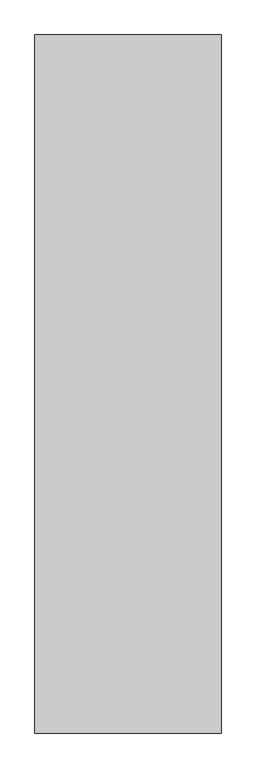
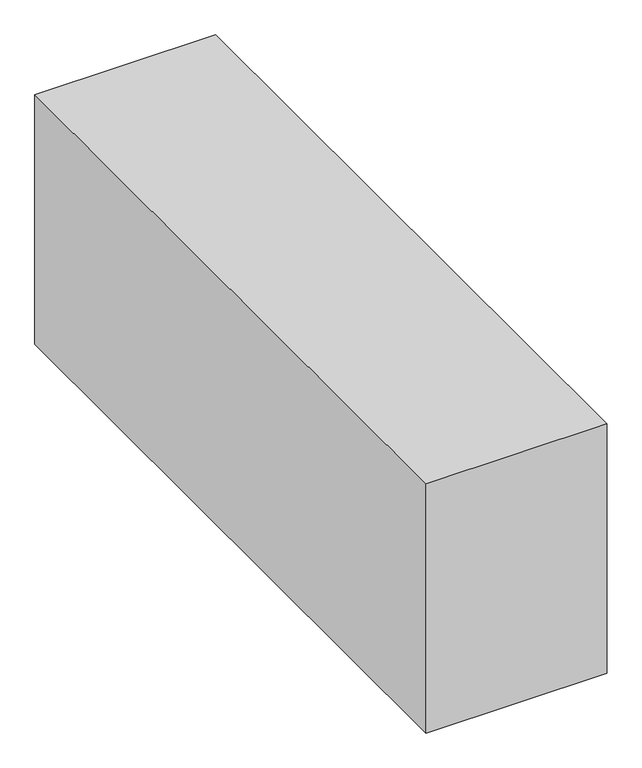
"""IFC4 building model written with IfcOpenShell, lengths in millimetres: proxy geometry, Space Planning Box_hec : Space Planning Box_hec."""

import ifcopenshell
import ifcopenshell.guid

model = None  # the IFC model being written
_history = None  # IfcOwnerHistory: only IFC2X3 demands one
_inside = {}  # id of a spatial element -> (the spatial element, [elements in it])
_under = {}  # id of a project, library or spatial element -> (it, [spatial elements below it])
_declared = {}  # id of a project -> (the project, [libraries it declares])
_typed = {}  # id of a type object -> (the type object, [elements of that type])
_made_of = {}  # id of a material, layer set ... -> (it, [elements and type objects made of it])


def new_model(schema):
    """Start an empty IFC model of exactly this schema.

    Asked for "IFC4X3", IfcOpenShell would pick the latest addendum, in which some entities
    have other attributes; the version numbers below select the first issue.
    IFC2X3 requires an IfcOwnerHistory on every rooted entity: one is made here for all.
    """
    global model, _history
    if schema == "IFC4X3":
        model = ifcopenshell.file(schema_version=(4, 3, 0, 0))
    else:
        model = ifcopenshell.file(schema=schema)
    _inside.clear()
    _under.clear()
    _declared.clear()
    _typed.clear()
    _made_of.clear()
    _history = None
    if model.schema == "IFC2X3":
        org = make("IfcOrganization", Name="unknown")
        user = make(
            "IfcPersonAndOrganization",
            ThePerson=make("IfcPerson", FamilyName="unknown"),
            TheOrganization=org,
        )
        app = make(
            "IfcApplication",
            ApplicationDeveloper=org,
            Version="unknown",
            ApplicationFullName="unknown",
            ApplicationIdentifier="unknown",
        )
        _history = make(
            "IfcOwnerHistory",
            OwningUser=user,
            OwningApplication=app,
            ChangeAction="ADDED",
            CreationDate=0,
        )
    return model


def make(cls, **values):
    """One entity of the class cls with the attributes given. An attribute that is None is left unset."""
    return model.create_entity(
        cls, **{name: value for name, value in values.items() if value is not None}
    )


def rooted(cls, **values):
    """An entity with a GlobalId (a new one), such as an element, a storey or a relation."""
    return make(cls, GlobalId=ifcopenshell.guid.new(), OwnerHistory=_history, **values)


def si_unit(unit_type, name, prefix=None):
    """IfcSIUnit, for example si_unit("LENGTHUNIT", "METRE", prefix="MILLI")."""
    return make("IfcSIUnit", UnitType=unit_type, Prefix=prefix, Name=name)


def assignment(units):
    """IfcUnitAssignment: the units of a project."""
    return None if units is None else make("IfcUnitAssignment", Units=units)


def point(xyz):
    """IfcCartesianPoint."""
    return None if xyz is None else make("IfcCartesianPoint", Coordinates=xyz)


def direction(xyz):
    """IfcDirection."""
    return None if xyz is None else make("IfcDirection", DirectionRatios=xyz)


def frame(location, z_axis=None, x_axis=None):
    """IfcAxis2Placement3D, a coordinate frame: its origin and axes. An axis left out is left unset."""
    return make(
        "IfcAxis2Placement3D",
        Location=point(location),
        Axis=direction(z_axis),
        RefDirection=direction(x_axis),
    )


def origin():
    """The frame at (0, 0, 0) with its axes left unset."""
    return frame((0.0, 0.0, 0.0))


def origin_with_axes():
    """The frame at (0, 0, 0) with the z axis (0, 0, 1) and the x axis (1, 0, 0) written out."""
    return frame((0.0, 0.0, 0.0), z_axis=(0.0, 0.0, 1.0), x_axis=(1.0, 0.0, 0.0))


def place(relative_to, where):
    """IfcLocalPlacement: puts the frame where relative to a parent placement (None: the world)."""
    return make(
        "IfcLocalPlacement", PlacementRelTo=relative_to, RelativePlacement=where
    )


def context(
    kind, dimensions, precision=None, world=None, true_north=None, identifier=None
):
    """IfcGeometricRepresentationContext, for example the 3D "Model" context."""
    return make(
        "IfcGeometricRepresentationContext",
        ContextIdentifier=identifier,
        ContextType=kind,
        CoordinateSpaceDimension=dimensions,
        Precision=precision,
        WorldCoordinateSystem=world,
        TrueNorth=true_north,
    )


def project(units=None, contexts=None):
    """IfcProject with its units and contexts."""
    return rooted(
        "IfcProject",
        Name="project",
        RepresentationContexts=contexts,
        UnitsInContext=assignment(units),
    )


def spatial(cls, under=None, at=None, **own):
    """A site, building, storey or space (cls), placed at a placement, below another one or the project."""
    s = rooted(cls, ObjectPlacement=at, **own)
    if under is not None:
        _under.setdefault(under.id(), (under, []))[1].append(s)
    return s


def polyline(points):
    """IfcPolyline through the points."""
    return make("IfcPolyline", Points=[point(p) for p in points])


def outline(outer, holes=None, kind="AREA"):
    """IfcArbitraryClosedProfileDef: a profile drawn as a closed curve; with holes, ...WithVoids."""
    if holes is None:
        return make("IfcArbitraryClosedProfileDef", ProfileType=kind, OuterCurve=outer)
    return make(
        "IfcArbitraryProfileDefWithVoids",
        ProfileType=kind,
        OuterCurve=outer,
        InnerCurves=holes,
    )


def extrude(swept, where, along, depth):
    """IfcExtrudedAreaSolid: the profile swept, set in the frame where, extruded along a direction by depth."""
    return make(
        "IfcExtrudedAreaSolid",
        SweptArea=swept,
        Position=where,
        ExtrudedDirection=direction(along),
        Depth=depth,
    )


def shape(context_of_items, identifier, shape_type, items):
    """IfcShapeRepresentation: the items that make up one representation, for example the "Body"."""
    return make(
        "IfcShapeRepresentation",
        ContextOfItems=context_of_items,
        RepresentationIdentifier=identifier,
        RepresentationType=shape_type,
        Items=items,
    )


def source(mapping_origin, context_of_items, identifier, shape_type, items):
    """IfcRepresentationMap: a shape defined once, which mapped items show again and again."""
    return make(
        "IfcRepresentationMap",
        MappingOrigin=mapping_origin,
        MappedRepresentation=shape(context_of_items, identifier, shape_type, items),
    )


def transform(
    local_origin,
    x_axis=None,
    y_axis=None,
    z_axis=None,
    scale=None,
    scale2=None,
    scale3=None,
    uniform=True,
):
    """IfcCartesianTransformationOperator3D, or its non-uniform kind. x_axis, y_axis, z_axis: its Axis1, 2, 3."""
    if uniform:
        return make(
            "IfcCartesianTransformationOperator3D",
            Axis1=direction(x_axis),
            Axis2=direction(y_axis),
            LocalOrigin=point(local_origin),
            Scale=scale,
            Axis3=direction(z_axis),
        )
    return make(
        "IfcCartesianTransformationOperator3DnonUniform",
        Axis1=direction(x_axis),
        Axis2=direction(y_axis),
        LocalOrigin=point(local_origin),
        Scale=scale,
        Axis3=direction(z_axis),
        Scale2=scale2,
        Scale3=scale3,
    )


def mapped(mapping_source, mapping_target):
    """IfcMappedItem: shows the shape of a source again, moved by a transform."""
    return make(
        "IfcMappedItem", MappingSource=mapping_source, MappingTarget=mapping_target
    )


def made_of(thing, what):
    """Note that an element or type object is made of a material, layer set ...; save() writes the relation."""
    if what is not None:
        _made_of.setdefault(what.id(), (what, []))[1].append(thing)
    return thing


def element(
    cls,
    number,
    at=None,
    inside=None,
    cuts=None,
    type_object=None,
    material=None,
    context=None,
    identifier="Body",
    shape_type=None,
    held_by="IfcProductDefinitionShape",
    body=None,
    shapes=None,
    **own,
):
    """One element of the class cls, such as IfcWall. Its Tag is "e" and its number.

    at: its placement. inside: the storey or other place that contains it. cuts: it is an
    opening in that element (IfcRelVoidsElement). A single representation is given by context,
    identifier, shape_type and body (its items); several are given by shapes. held_by: the class
    of the entity that holds the representations. save() writes the other relations.
    """
    e = rooted(cls, Tag="e%d" % number, ObjectPlacement=at, **own)
    if body is not None:
        shapes = [shape(context, identifier, shape_type, body)]
    if shapes is not None:
        e.Representation = make(held_by, Representations=shapes)
    if inside is not None:
        _inside.setdefault(inside.id(), (inside, []))[1].append(e)
    if cuts is not None:
        rooted(
            "IfcRelVoidsElement", RelatingBuildingElement=cuts, RelatedOpeningElement=e
        )
    if type_object is not None:
        _typed.setdefault(type_object.id(), (type_object, []))[1].append(e)
    return made_of(e, material)


def aggregate(whole, parts):
    """IfcRelAggregates: a whole, such as a stair, and the parts it consists of."""
    return rooted("IfcRelAggregates", RelatingObject=whole, RelatedObjects=parts)


def save(model, path):
    """Write the relations noted so far, then the file.

    IfcRelAggregates (storeys below a building ...), IfcRelContainedInSpatialStructure (elements
    in a storey), IfcRelDefinesByType, IfcRelAssociatesMaterial and IfcRelDeclares: one each for
    every whole, place, type object, material and project.
    """
    for whole, parts in _under.values():
        aggregate(whole, parts)
    for where, things in _inside.values():
        rooted(
            "IfcRelContainedInSpatialStructure",
            RelatedElements=things,
            RelatingStructure=where,
        )
    for kind, things in _typed.values():
        rooted("IfcRelDefinesByType", RelatedObjects=things, RelatingType=kind)
    for what, things in _made_of.values():
        rooted("IfcRelAssociatesMaterial", RelatedObjects=things, RelatingMaterial=what)
    for by, libraries in _declared.values():
        rooted("IfcRelDeclares", RelatingContext=by, RelatedDefinitions=libraries)
    model.write(path)


def generic_models_3f6e5246(model_context):
    return source(origin(), model_context, "Body", "SweptSolid", [
        extrude(outline(polyline([(1200.0, 4500.0), (1200.0, -4500.0), (-1200.0, -4500.0), (-1200.0, 4500.0), (1200.0, 4500.0)])), origin_with_axes(), (0.0, 0.0, 1.0), 3500.0),
    ])


if __name__ == "__main__":
    model = new_model("IFC4")
    model_context = context("Model", 3, world=origin())
    ifc_project = project(units=[si_unit("LENGTHUNIT", "METRE", prefix="MILLI")], contexts=[model_context])
    site = spatial("IfcSite", under=ifc_project)
    building = spatial("IfcBuilding", under=site)
    placement = place(None, origin())
    generic_models_shape = generic_models_3f6e5246(model_context)
    element("IfcBuildingElementProxy", 1, Name="Space Planning Box_hec : Space Planning Box_hec", ObjectType="Space Planning Box_hec : Space Planning Box_hec", at=placement, inside=building, context=model_context, shape_type="MappedRepresentation", body=[
        mapped(generic_models_shape, transform((0.0, 0.0, 0.0), x_axis=(1.0, 0.0, 0.0), y_axis=(0.0, 1.0, 0.0), z_axis=(0.0, 0.0, 1.0))),
    ])
    save(model, "model.ifc")

# Revit data of these elements
# Project information
#   Building Name = "MAIN GATE SECURITY BUILDING"
#   Project Status = "Project Status"
#   Client Name = "현대엔지니어링"
#   Project Address = "서울시 종로구 율곡로 75(계동)"
#   Project Name = "Therma Visayas Energy Project"
#   Project Number = "-"
# Type "Space Planning Box_hec : Space Planning Box_hec"
#   Type Comments = "..."
#   Room Name [instance default] = "?"
#   Interior Finish [instance default] = ""
#   Exterior Finish [instance default] = ""
#   Department [instance default] = ""
#   Assembly Code = "..."
#   ceiling height [instance default] = 0
#   Width [instance default] = 1524 mm
#   Program Area [instance default] = 0.00 m²
#   Length [instance default] = 1524 mm
#   Height [instance default] = 1524 mm
#   Area [instance default] = 2.32258 m²
#   Fill Color [instance default] = Cyan
#   Default Elevation = 0
# Element 1 (IfcBuildingElementProxy, "Space Planning Box_hec : Space Planning Box_hec")
#   Room Name = "Duct Shaft"
#   Exterior Finish = "RF1..N/A,,EW2..N/A..N/A"
#   Department = "PATHV3"
#   Width = 2400 mm
#   Program Area = 21.60 m²
#   Length = 9000 mm
#   Height = 3500 mm
#   Area = 21.60 m²
#   Fill Color = Lavender
#   Materials on its faces: "Lavender"
# Materials
#   "Cyan": class "Generic", colour RGB 0 255 255, transparency 0.2, Cost = 0
#   "Lavender": class "Generic", colour RGB 186 85 211, transparency 0.2, Cost = 0
